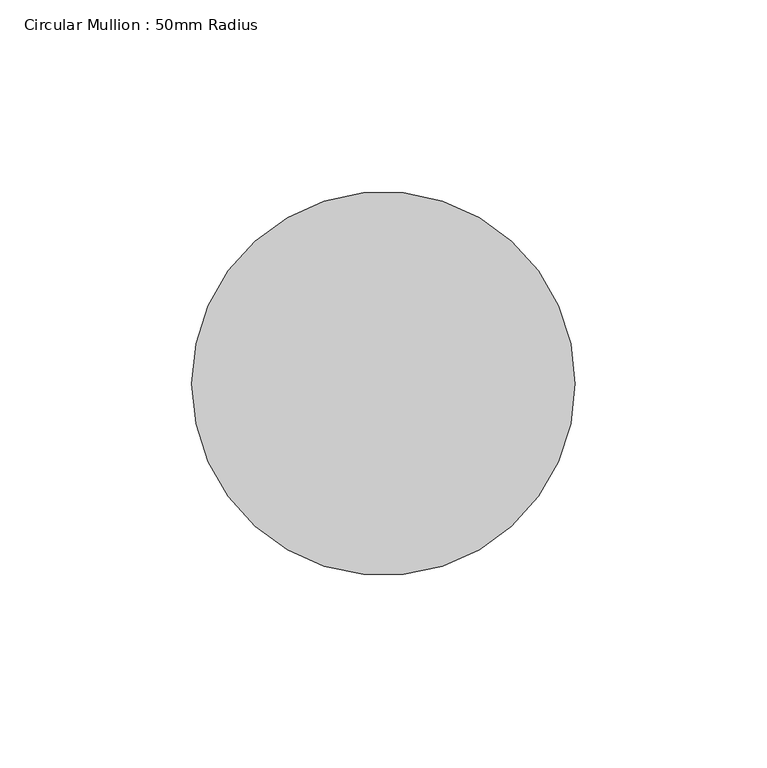
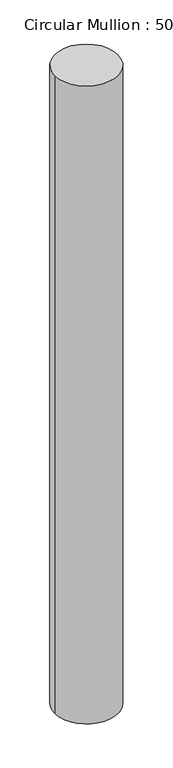
"""IFC4 building model written with IfcOpenShell, lengths in millimetres: member geometry, Circular Mullion : 50mm Radius."""

from ifc_helpers import new_model, si_unit, point, frame, origin, origin_2d, place, context, project, spatial, circle_curve, trimmed, segment, composite_curve, outline, extrude, source, transform, mapped, element, save


def circular_mullion_50mm_radius_3da2af72(model_context):
    return source(origin(), model_context, "Body", "SweptSolid", [
        extrude(outline(composite_curve([segment(trimmed(circle_curve(origin_2d(), 50.0), [point((50.0, 0.0))], [point((-50.0, 0.0))], False, "CARTESIAN"), True, "CONTINUOUS"), segment(trimmed(circle_curve(origin_2d(), 50.0), [point((-50.0, 0.0))], [point((50.0, 0.0))], False, "CARTESIAN"), True, "CONTINUOUS")], self_intersect=False)), frame((0.0, 0.0, -1067.4692499), z_axis=(0.0, 0.0, 1.0), x_axis=(1.0, 0.0, 0.0)), (0.0, 0.0, 1.0), 1067.4692499),
    ])


if __name__ == "__main__":
    model = new_model("IFC4")
    model_context = context("Model", 3, world=origin())
    ifc_project = project(units=[si_unit("LENGTHUNIT", "METRE", prefix="MILLI")], contexts=[model_context])
    site = spatial("IfcSite", under=ifc_project)
    building = spatial("IfcBuilding", under=site)
    placement = place(None, origin())
    circular_mullion_50mm_radius_shape = circular_mullion_50mm_radius_3da2af72(model_context)
    element("IfcMember", 1, ObjectType="Circular Mullion : 50mm Radius", at=placement, inside=building, context=model_context, shape_type="MappedRepresentation", body=[
        mapped(circular_mullion_50mm_radius_shape, transform((0.0, 0.0, 0.0), x_axis=(1.0, 0.0, 0.0), y_axis=(0.0, 1.0, 0.0), z_axis=(0.0, 0.0, 1.0))),
    ])
    save(model, "model.ifc")

# Revit data of these elements
# Type "Circular Mullion : 50mm Radius"
#   built-in parameter 1007350 = 0.164042 (stored number, unit not read)
# Element 1 (IfcMember, "Circular Mullion : 50mm Radius")
#   Materials on its faces: "Aluminium"
# Materials
#   "Aluminium": class "Metal", colour RGB 247 247 247, transparency 0, Description = "Aluminium 6061", Cost = 0
